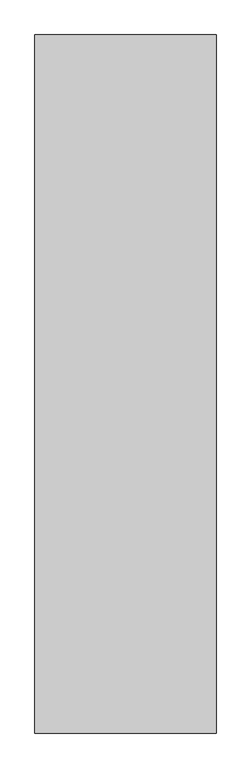
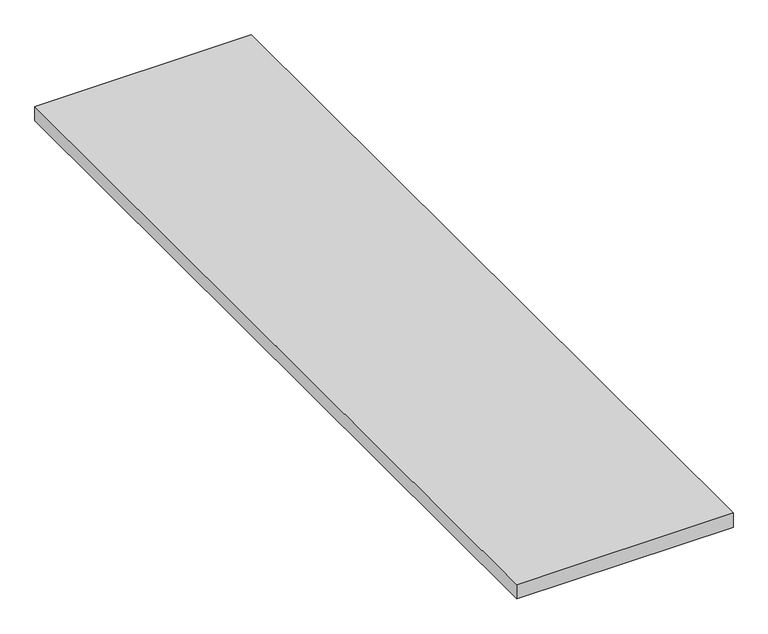
"""IFC4 building model written with IfcOpenShell, lengths in millimetres: proxy geometry, Flooring005 668 : Flooring005 668."""

from ifc_helpers import new_model, si_unit, frame, origin, place, context, project, spatial, polyline, outline, extrude, source, transform, mapped, element, save


def generic_models_d10a6021(model_context):
    return source(origin(), model_context, "Body", "SweptSolid", [
        extrude(outline(polyline([(-6524.519043, 7982.1531721), (-7043.5268555, 7982.1531721), (-7043.5268555, 9982.1531721), (-6524.519043, 9982.1531721), (-6524.519043, 7982.1531721)])), frame((0.0, 0.0, 40171.0155395), z_axis=(0.0, 0.0, 1.0), x_axis=(1.0, 0.0, 0.0)), (0.0, 0.0, 1.0), 35.7929688),
    ])


if __name__ == "__main__":
    model = new_model("IFC4")
    model_context = context("Model", 3, world=origin())
    ifc_project = project(units=[si_unit("LENGTHUNIT", "METRE", prefix="MILLI")], contexts=[model_context])
    site = spatial("IfcSite", under=ifc_project)
    building = spatial("IfcBuilding", under=site)
    placement = place(None, origin())
    generic_models_shape = generic_models_d10a6021(model_context)
    element("IfcBuildingElementProxy", 1, Name="Flooring005 668 : Flooring005 668", ObjectType="Flooring005 668 : Flooring005 668", at=placement, inside=building, context=model_context, shape_type="MappedRepresentation", body=[
        mapped(generic_models_shape, transform((0.0, 0.0, 0.0), x_axis=(1.0, 0.0, 0.0), y_axis=(0.0, 1.0, 0.0), z_axis=(0.0, 0.0, 1.0))),
    ])
    save(model, "model.ifc")

# Revit data of these elements
# Type "Flooring005 668 : Flooring005 668"
#   NameOverride = "Flooring005"
# Element 1 (IfcBuildingElementProxy, "Flooring005 668 : Flooring005 668")
#   Materials on its faces: "TERRACE FLOORING TBD"
# Materials
#   "TERRACE FLOORING TBD": class "Unassigned", colour RGB 128 128 128, transparency 0
